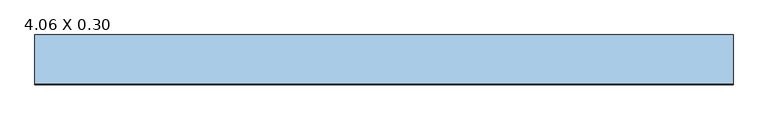
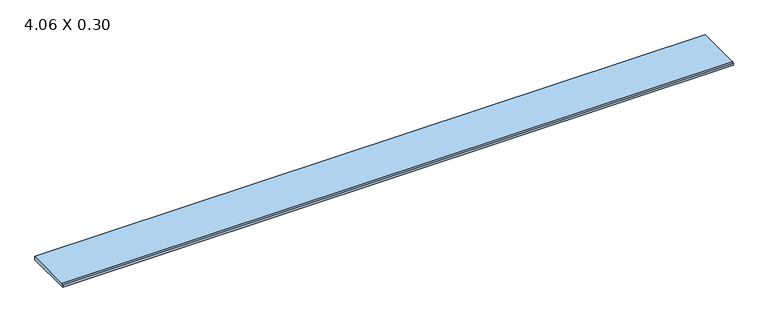
"""IFC4 building model written with IfcOpenShell, lengths in millimetres: window geometry, .CC_ND 300_PEDRA_PEITORIL RETO : 4.06 X 0.30."""

import ifcopenshell
import ifcopenshell.guid

model = None  # the IFC model being written
_history = None  # IfcOwnerHistory: only IFC2X3 demands one
_inside = {}  # id of a spatial element -> (the spatial element, [elements in it])
_under = {}  # id of a project, library or spatial element -> (it, [spatial elements below it])
_declared = {}  # id of a project -> (the project, [libraries it declares])
_typed = {}  # id of a type object -> (the type object, [elements of that type])
_made_of = {}  # id of a material, layer set ... -> (it, [elements and type objects made of it])


def new_model(schema):
    """Start an empty IFC model of exactly this schema.

    Asked for "IFC4X3", IfcOpenShell would pick the latest addendum, in which some entities
    have other attributes; the version numbers below select the first issue.
    IFC2X3 requires an IfcOwnerHistory on every rooted entity: one is made here for all.
    """
    global model, _history
    if schema == "IFC4X3":
        model = ifcopenshell.file(schema_version=(4, 3, 0, 0))
    else:
        model = ifcopenshell.file(schema=schema)
    _inside.clear()
    _under.clear()
    _declared.clear()
    _typed.clear()
    _made_of.clear()
    _history = None
    if model.schema == "IFC2X3":
        org = make("IfcOrganization", Name="unknown")
        user = make(
            "IfcPersonAndOrganization",
            ThePerson=make("IfcPerson", FamilyName="unknown"),
            TheOrganization=org,
        )
        app = make(
            "IfcApplication",
            ApplicationDeveloper=org,
            Version="unknown",
            ApplicationFullName="unknown",
            ApplicationIdentifier="unknown",
        )
        _history = make(
            "IfcOwnerHistory",
            OwningUser=user,
            OwningApplication=app,
            ChangeAction="ADDED",
            CreationDate=0,
        )
    return model


def make(cls, **values):
    """One entity of the class cls with the attributes given. An attribute that is None is left unset."""
    return model.create_entity(
        cls, **{name: value for name, value in values.items() if value is not None}
    )


def rooted(cls, **values):
    """An entity with a GlobalId (a new one), such as an element, a storey or a relation."""
    return make(cls, GlobalId=ifcopenshell.guid.new(), OwnerHistory=_history, **values)


def si_unit(unit_type, name, prefix=None):
    """IfcSIUnit, for example si_unit("LENGTHUNIT", "METRE", prefix="MILLI")."""
    return make("IfcSIUnit", UnitType=unit_type, Prefix=prefix, Name=name)


def assignment(units):
    """IfcUnitAssignment: the units of a project."""
    return None if units is None else make("IfcUnitAssignment", Units=units)


def point(xyz):
    """IfcCartesianPoint."""
    return None if xyz is None else make("IfcCartesianPoint", Coordinates=xyz)


def direction(xyz):
    """IfcDirection."""
    return None if xyz is None else make("IfcDirection", DirectionRatios=xyz)


def frame(location, z_axis=None, x_axis=None):
    """IfcAxis2Placement3D, a coordinate frame: its origin and axes. An axis left out is left unset."""
    return make(
        "IfcAxis2Placement3D",
        Location=point(location),
        Axis=direction(z_axis),
        RefDirection=direction(x_axis),
    )


def frame_2d(location, x_axis=None):
    """IfcAxis2Placement2D, a coordinate frame in the plane: its origin and x axis."""
    return make(
        "IfcAxis2Placement2D", Location=point(location), RefDirection=direction(x_axis)
    )


def origin():
    """The frame at (0, 0, 0) with its axes left unset."""
    return frame((0.0, 0.0, 0.0))


def place(relative_to, where):
    """IfcLocalPlacement: puts the frame where relative to a parent placement (None: the world)."""
    return make(
        "IfcLocalPlacement", PlacementRelTo=relative_to, RelativePlacement=where
    )


def context(
    kind, dimensions, precision=None, world=None, true_north=None, identifier=None
):
    """IfcGeometricRepresentationContext, for example the 3D "Model" context."""
    return make(
        "IfcGeometricRepresentationContext",
        ContextIdentifier=identifier,
        ContextType=kind,
        CoordinateSpaceDimension=dimensions,
        Precision=precision,
        WorldCoordinateSystem=world,
        TrueNorth=true_north,
    )


def project(units=None, contexts=None):
    """IfcProject with its units and contexts."""
    return rooted(
        "IfcProject",
        Name="project",
        RepresentationContexts=contexts,
        UnitsInContext=assignment(units),
    )


def spatial(cls, under=None, at=None, **own):
    """A site, building, storey or space (cls), placed at a placement, below another one or the project."""
    s = rooted(cls, ObjectPlacement=at, **own)
    if under is not None:
        _under.setdefault(under.id(), (under, []))[1].append(s)
    return s


def polyline(points):
    """IfcPolyline through the points."""
    return make("IfcPolyline", Points=[point(p) for p in points])


def circle_curve(where, radius):
    """IfcCircle in the frame where."""
    return make("IfcCircle", Position=where, Radius=radius)


def trimmed(basis, trim1, trim2, sense, master):
    """IfcTrimmedCurve: the piece of a basis curve between two trims."""
    return make(
        "IfcTrimmedCurve",
        BasisCurve=basis,
        Trim1=trim1,
        Trim2=trim2,
        SenseAgreement=sense,
        MasterRepresentation=master,
    )


def segment(curve, same_sense, transition):
    """IfcCompositeCurveSegment."""
    return make(
        "IfcCompositeCurveSegment",
        Transition=transition,
        SameSense=same_sense,
        ParentCurve=curve,
    )


def composite_curve(segments, self_intersect=None):
    """IfcCompositeCurve: segments joined end to end."""
    return make("IfcCompositeCurve", Segments=segments, SelfIntersect=self_intersect)


def outline(outer, holes=None, kind="AREA"):
    """IfcArbitraryClosedProfileDef: a profile drawn as a closed curve; with holes, ...WithVoids."""
    if holes is None:
        return make("IfcArbitraryClosedProfileDef", ProfileType=kind, OuterCurve=outer)
    return make(
        "IfcArbitraryProfileDefWithVoids",
        ProfileType=kind,
        OuterCurve=outer,
        InnerCurves=holes,
    )


def extrude(swept, where, along, depth):
    """IfcExtrudedAreaSolid: the profile swept, set in the frame where, extruded along a direction by depth."""
    return make(
        "IfcExtrudedAreaSolid",
        SweptArea=swept,
        Position=where,
        ExtrudedDirection=direction(along),
        Depth=depth,
    )


def shape(context_of_items, identifier, shape_type, items):
    """IfcShapeRepresentation: the items that make up one representation, for example the "Body"."""
    return make(
        "IfcShapeRepresentation",
        ContextOfItems=context_of_items,
        RepresentationIdentifier=identifier,
        RepresentationType=shape_type,
        Items=items,
    )


def source(mapping_origin, context_of_items, identifier, shape_type, items):
    """IfcRepresentationMap: a shape defined once, which mapped items show again and again."""
    return make(
        "IfcRepresentationMap",
        MappingOrigin=mapping_origin,
        MappedRepresentation=shape(context_of_items, identifier, shape_type, items),
    )


def transform(
    local_origin,
    x_axis=None,
    y_axis=None,
    z_axis=None,
    scale=None,
    scale2=None,
    scale3=None,
    uniform=True,
):
    """IfcCartesianTransformationOperator3D, or its non-uniform kind. x_axis, y_axis, z_axis: its Axis1, 2, 3."""
    if uniform:
        return make(
            "IfcCartesianTransformationOperator3D",
            Axis1=direction(x_axis),
            Axis2=direction(y_axis),
            LocalOrigin=point(local_origin),
            Scale=scale,
            Axis3=direction(z_axis),
        )
    return make(
        "IfcCartesianTransformationOperator3DnonUniform",
        Axis1=direction(x_axis),
        Axis2=direction(y_axis),
        LocalOrigin=point(local_origin),
        Scale=scale,
        Axis3=direction(z_axis),
        Scale2=scale2,
        Scale3=scale3,
    )


def mapped(mapping_source, mapping_target):
    """IfcMappedItem: shows the shape of a source again, moved by a transform."""
    return make(
        "IfcMappedItem", MappingSource=mapping_source, MappingTarget=mapping_target
    )


def made_of(thing, what):
    """Note that an element or type object is made of a material, layer set ...; save() writes the relation."""
    if what is not None:
        _made_of.setdefault(what.id(), (what, []))[1].append(thing)
    return thing


def element(
    cls,
    number,
    at=None,
    inside=None,
    cuts=None,
    type_object=None,
    material=None,
    context=None,
    identifier="Body",
    shape_type=None,
    held_by="IfcProductDefinitionShape",
    body=None,
    shapes=None,
    **own,
):
    """One element of the class cls, such as IfcWall. Its Tag is "e" and its number.

    at: its placement. inside: the storey or other place that contains it. cuts: it is an
    opening in that element (IfcRelVoidsElement). A single representation is given by context,
    identifier, shape_type and body (its items); several are given by shapes. held_by: the class
    of the entity that holds the representations. save() writes the other relations.
    """
    e = rooted(cls, Tag="e%d" % number, ObjectPlacement=at, **own)
    if body is not None:
        shapes = [shape(context, identifier, shape_type, body)]
    if shapes is not None:
        e.Representation = make(held_by, Representations=shapes)
    if inside is not None:
        _inside.setdefault(inside.id(), (inside, []))[1].append(e)
    if cuts is not None:
        rooted(
            "IfcRelVoidsElement", RelatingBuildingElement=cuts, RelatedOpeningElement=e
        )
    if type_object is not None:
        _typed.setdefault(type_object.id(), (type_object, []))[1].append(e)
    return made_of(e, material)


def aggregate(whole, parts):
    """IfcRelAggregates: a whole, such as a stair, and the parts it consists of."""
    return rooted("IfcRelAggregates", RelatingObject=whole, RelatedObjects=parts)


def save(model, path):
    """Write the relations noted so far, then the file.

    IfcRelAggregates (storeys below a building ...), IfcRelContainedInSpatialStructure (elements
    in a storey), IfcRelDefinesByType, IfcRelAssociatesMaterial and IfcRelDeclares: one each for
    every whole, place, type object, material and project.
    """
    for whole, parts in _under.values():
        aggregate(whole, parts)
    for where, things in _inside.values():
        rooted(
            "IfcRelContainedInSpatialStructure",
            RelatedElements=things,
            RelatingStructure=where,
        )
    for kind, things in _typed.values():
        rooted("IfcRelDefinesByType", RelatedObjects=things, RelatingType=kind)
    for what, things in _made_of.values():
        rooted("IfcRelAssociatesMaterial", RelatedObjects=things, RelatingMaterial=what)
    for by, libraries in _declared.values():
        rooted("IfcRelDeclares", RelatingContext=by, RelatedDefinitions=libraries)
    model.write(path)


def window_4_06_x_0_30_b1d56b02(model_context):
    return source(origin(), model_context, "Body", "SweptSolid", [
        extrude(outline(composite_curve([segment(polyline([(-144.4083081, 1480.0), (-144.4083081, 1488.1993124), (-149.1619526, 1488.1993124), (-149.1619526, 1480.0), (-159.9, 1480.0), (-159.9, 1493.3808343)]), True, "CONTINUOUS"), segment(trimmed(circle_curve(frame_2d((-153.2808343, 1493.3808343)), 6.6191657), [point((-159.9, 1493.3808343))], [point((-153.2808343, 1500.0))], False, "CARTESIAN"), True, "CONTINUOUS"), segment(polyline([(-153.2808343, 1500.0), (129.9, 1500.0), (129.9, 1480.0), (-144.4083081, 1480.0)]), True, "CONTINUOUS")], self_intersect=False)), frame((-2030.0, 0.0, 0.0), z_axis=(1.0, 0.0, 0.0), x_axis=(0.0, 1.0, 0.0)), (0.0, 0.0, 1.0), 4060.0),
    ])


if __name__ == "__main__":
    model = new_model("IFC4")
    model_context = context("Model", 3, world=origin())
    ifc_project = project(units=[si_unit("LENGTHUNIT", "METRE", prefix="MILLI")], contexts=[model_context])
    site = spatial("IfcSite", under=ifc_project)
    building = spatial("IfcBuilding", under=site)
    placement = place(None, origin())
    window_4_06_x_0_30_shape = window_4_06_x_0_30_b1d56b02(model_context)
    element("IfcWindow", 1, ObjectType=".CC_ND 300_PEDRA_PEITORIL RETO : 4.06 X 0.30", at=placement, inside=building, context=model_context, shape_type="MappedRepresentation", body=[
        mapped(window_4_06_x_0_30_shape, transform((0.0, 0.0, 0.0), x_axis=(1.0, 0.0, 0.0), y_axis=(0.0, 1.0, 0.0), z_axis=(0.0, 0.0, 1.0))),
    ])
    save(model, "model.ifc")

# Revit data of these elements
# Type ".CC_ND 300_PEDRA_PEITORIL RETO : 4.06 X 0.30"
#   Type Mark = "72"
#   Largura da pedra [instance default] = 0.26 m
#   Extensão interior peitoril [instance default] = 0.03 m
#   Extensão exterior peitoril [instance default] = 0.03 m
#   Espessura = 0.02 m
#   Comprimento = 4.06 m
#   Altura-padrão do peitoril = 1.48 m
#   Peitoril = .GRANITO_BRANCO_ITAUNAS
#   Rough Width = 0
#   Rough Height = 0
#   Height = 0
#   Wall Closure = (empty or 0)
#   Width = 0
# Element 1 (IfcWindow, ".CC_ND 300_PEDRA_PEITORIL RETO : 4.06 X 0.30")
#   Largura da pedra = 0.2898 m
#   Extensão interior peitoril = 0.00 m
#   Materials on its faces: ".GRANITO_BRANCO_ITAUNAS"
# Materials
#   ".GRANITO_BRANCO_ITAUNAS": class ".CC_PEDRA REVEST.", colour RGB 202 195 174, transparency 0, Description = "Revestimento em granito", Cost = 0
